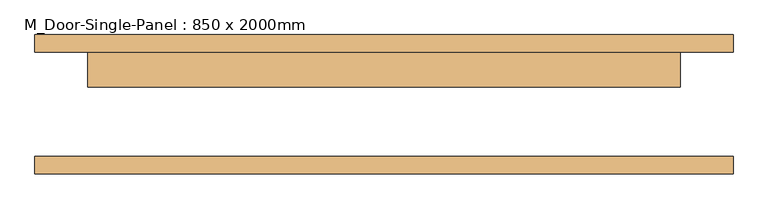
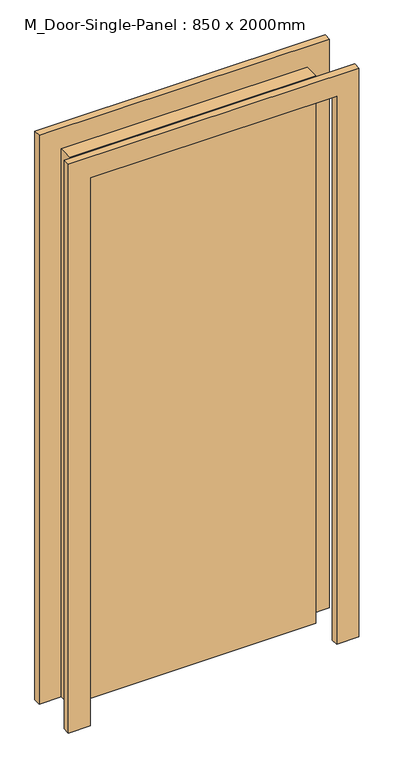
"""IFC4 building model written with IfcOpenShell, lengths in millimetres: door geometry, M_Door-Single-Panel : 850 x 2000mm."""

import ifcopenshell
import ifcopenshell.guid

model = None  # the IFC model being written
_history = None  # IfcOwnerHistory: only IFC2X3 demands one
_inside = {}  # id of a spatial element -> (the spatial element, [elements in it])
_under = {}  # id of a project, library or spatial element -> (it, [spatial elements below it])
_declared = {}  # id of a project -> (the project, [libraries it declares])
_typed = {}  # id of a type object -> (the type object, [elements of that type])
_made_of = {}  # id of a material, layer set ... -> (it, [elements and type objects made of it])


def new_model(schema):
    """Start an empty IFC model of exactly this schema.

    Asked for "IFC4X3", IfcOpenShell would pick the latest addendum, in which some entities
    have other attributes; the version numbers below select the first issue.
    IFC2X3 requires an IfcOwnerHistory on every rooted entity: one is made here for all.
    """
    global model, _history
    if schema == "IFC4X3":
        model = ifcopenshell.file(schema_version=(4, 3, 0, 0))
    else:
        model = ifcopenshell.file(schema=schema)
    _inside.clear()
    _under.clear()
    _declared.clear()
    _typed.clear()
    _made_of.clear()
    _history = None
    if model.schema == "IFC2X3":
        org = make("IfcOrganization", Name="unknown")
        user = make(
            "IfcPersonAndOrganization",
            ThePerson=make("IfcPerson", FamilyName="unknown"),
            TheOrganization=org,
        )
        app = make(
            "IfcApplication",
            ApplicationDeveloper=org,
            Version="unknown",
            ApplicationFullName="unknown",
            ApplicationIdentifier="unknown",
        )
        _history = make(
            "IfcOwnerHistory",
            OwningUser=user,
            OwningApplication=app,
            ChangeAction="ADDED",
            CreationDate=0,
        )
    return model


def make(cls, **values):
    """One entity of the class cls with the attributes given. An attribute that is None is left unset."""
    return model.create_entity(
        cls, **{name: value for name, value in values.items() if value is not None}
    )


def rooted(cls, **values):
    """An entity with a GlobalId (a new one), such as an element, a storey or a relation."""
    return make(cls, GlobalId=ifcopenshell.guid.new(), OwnerHistory=_history, **values)


def si_unit(unit_type, name, prefix=None):
    """IfcSIUnit, for example si_unit("LENGTHUNIT", "METRE", prefix="MILLI")."""
    return make("IfcSIUnit", UnitType=unit_type, Prefix=prefix, Name=name)


def assignment(units):
    """IfcUnitAssignment: the units of a project."""
    return None if units is None else make("IfcUnitAssignment", Units=units)


def point(xyz):
    """IfcCartesianPoint."""
    return None if xyz is None else make("IfcCartesianPoint", Coordinates=xyz)


def direction(xyz):
    """IfcDirection."""
    return None if xyz is None else make("IfcDirection", DirectionRatios=xyz)


def frame(location, z_axis=None, x_axis=None):
    """IfcAxis2Placement3D, a coordinate frame: its origin and axes. An axis left out is left unset."""
    return make(
        "IfcAxis2Placement3D",
        Location=point(location),
        Axis=direction(z_axis),
        RefDirection=direction(x_axis),
    )


def origin():
    """The frame at (0, 0, 0) with its axes left unset."""
    return frame((0.0, 0.0, 0.0))


def origin_with_axes():
    """The frame at (0, 0, 0) with the z axis (0, 0, 1) and the x axis (1, 0, 0) written out."""
    return frame((0.0, 0.0, 0.0), z_axis=(0.0, 0.0, 1.0), x_axis=(1.0, 0.0, 0.0))


def place(relative_to, where):
    """IfcLocalPlacement: puts the frame where relative to a parent placement (None: the world)."""
    return make(
        "IfcLocalPlacement", PlacementRelTo=relative_to, RelativePlacement=where
    )


def context(
    kind, dimensions, precision=None, world=None, true_north=None, identifier=None
):
    """IfcGeometricRepresentationContext, for example the 3D "Model" context."""
    return make(
        "IfcGeometricRepresentationContext",
        ContextIdentifier=identifier,
        ContextType=kind,
        CoordinateSpaceDimension=dimensions,
        Precision=precision,
        WorldCoordinateSystem=world,
        TrueNorth=true_north,
    )


def project(units=None, contexts=None):
    """IfcProject with its units and contexts."""
    return rooted(
        "IfcProject",
        Name="project",
        RepresentationContexts=contexts,
        UnitsInContext=assignment(units),
    )


def spatial(cls, under=None, at=None, **own):
    """A site, building, storey or space (cls), placed at a placement, below another one or the project."""
    s = rooted(cls, ObjectPlacement=at, **own)
    if under is not None:
        _under.setdefault(under.id(), (under, []))[1].append(s)
    return s


def polyline(points):
    """IfcPolyline through the points."""
    return make("IfcPolyline", Points=[point(p) for p in points])


def outline(outer, holes=None, kind="AREA"):
    """IfcArbitraryClosedProfileDef: a profile drawn as a closed curve; with holes, ...WithVoids."""
    if holes is None:
        return make("IfcArbitraryClosedProfileDef", ProfileType=kind, OuterCurve=outer)
    return make(
        "IfcArbitraryProfileDefWithVoids",
        ProfileType=kind,
        OuterCurve=outer,
        InnerCurves=holes,
    )


def extrude(swept, where, along, depth):
    """IfcExtrudedAreaSolid: the profile swept, set in the frame where, extruded along a direction by depth."""
    return make(
        "IfcExtrudedAreaSolid",
        SweptArea=swept,
        Position=where,
        ExtrudedDirection=direction(along),
        Depth=depth,
    )


def shape(context_of_items, identifier, shape_type, items):
    """IfcShapeRepresentation: the items that make up one representation, for example the "Body"."""
    return make(
        "IfcShapeRepresentation",
        ContextOfItems=context_of_items,
        RepresentationIdentifier=identifier,
        RepresentationType=shape_type,
        Items=items,
    )


def source(mapping_origin, context_of_items, identifier, shape_type, items):
    """IfcRepresentationMap: a shape defined once, which mapped items show again and again."""
    return make(
        "IfcRepresentationMap",
        MappingOrigin=mapping_origin,
        MappedRepresentation=shape(context_of_items, identifier, shape_type, items),
    )


def transform(
    local_origin,
    x_axis=None,
    y_axis=None,
    z_axis=None,
    scale=None,
    scale2=None,
    scale3=None,
    uniform=True,
):
    """IfcCartesianTransformationOperator3D, or its non-uniform kind. x_axis, y_axis, z_axis: its Axis1, 2, 3."""
    if uniform:
        return make(
            "IfcCartesianTransformationOperator3D",
            Axis1=direction(x_axis),
            Axis2=direction(y_axis),
            LocalOrigin=point(local_origin),
            Scale=scale,
            Axis3=direction(z_axis),
        )
    return make(
        "IfcCartesianTransformationOperator3DnonUniform",
        Axis1=direction(x_axis),
        Axis2=direction(y_axis),
        LocalOrigin=point(local_origin),
        Scale=scale,
        Axis3=direction(z_axis),
        Scale2=scale2,
        Scale3=scale3,
    )


def mapped(mapping_source, mapping_target):
    """IfcMappedItem: shows the shape of a source again, moved by a transform."""
    return make(
        "IfcMappedItem", MappingSource=mapping_source, MappingTarget=mapping_target
    )


def made_of(thing, what):
    """Note that an element or type object is made of a material, layer set ...; save() writes the relation."""
    if what is not None:
        _made_of.setdefault(what.id(), (what, []))[1].append(thing)
    return thing


def element(
    cls,
    number,
    at=None,
    inside=None,
    cuts=None,
    type_object=None,
    material=None,
    context=None,
    identifier="Body",
    shape_type=None,
    held_by="IfcProductDefinitionShape",
    body=None,
    shapes=None,
    **own,
):
    """One element of the class cls, such as IfcWall. Its Tag is "e" and its number.

    at: its placement. inside: the storey or other place that contains it. cuts: it is an
    opening in that element (IfcRelVoidsElement). A single representation is given by context,
    identifier, shape_type and body (its items); several are given by shapes. held_by: the class
    of the entity that holds the representations. save() writes the other relations.
    """
    e = rooted(cls, Tag="e%d" % number, ObjectPlacement=at, **own)
    if body is not None:
        shapes = [shape(context, identifier, shape_type, body)]
    if shapes is not None:
        e.Representation = make(held_by, Representations=shapes)
    if inside is not None:
        _inside.setdefault(inside.id(), (inside, []))[1].append(e)
    if cuts is not None:
        rooted(
            "IfcRelVoidsElement", RelatingBuildingElement=cuts, RelatedOpeningElement=e
        )
    if type_object is not None:
        _typed.setdefault(type_object.id(), (type_object, []))[1].append(e)
    return made_of(e, material)


def aggregate(whole, parts):
    """IfcRelAggregates: a whole, such as a stair, and the parts it consists of."""
    return rooted("IfcRelAggregates", RelatingObject=whole, RelatedObjects=parts)


def save(model, path):
    """Write the relations noted so far, then the file.

    IfcRelAggregates (storeys below a building ...), IfcRelContainedInSpatialStructure (elements
    in a storey), IfcRelDefinesByType, IfcRelAssociatesMaterial and IfcRelDeclares: one each for
    every whole, place, type object, material and project.
    """
    for whole, parts in _under.values():
        aggregate(whole, parts)
    for where, things in _inside.values():
        rooted(
            "IfcRelContainedInSpatialStructure",
            RelatedElements=things,
            RelatingStructure=where,
        )
    for kind, things in _typed.values():
        rooted("IfcRelDefinesByType", RelatedObjects=things, RelatingType=kind)
    for what, things in _made_of.values():
        rooted("IfcRelAssociatesMaterial", RelatedObjects=things, RelatingMaterial=what)
    for by, libraries in _declared.values():
        rooted("IfcRelDeclares", RelatingContext=by, RelatedDefinitions=libraries)
    model.write(path)


def m_door_single_panel_850_x_2000mm_c4dca14f(model_context):
    return source(origin(), model_context, "Body", "SweptSolid", [
        extrude(outline(polyline([(425.0, 25.0), (-425.0, 25.0), (-425.0, 75.0), (425.0, 75.0), (425.0, 25.0)])), origin_with_axes(), (0.0, 0.0, 1.0), 2000.0),
        extrude(outline(polyline([(2076.2, -501.2), (0.0, -501.2), (0.0, -425.0), (2000.0, -425.0), (2000.0, 425.0), (0.0, 425.0), (0.0, 501.2), (2076.2, 501.2), (2076.2, -501.2)])), frame((0.0, 75.0, 0.0), z_axis=(0.0, 1.0, 0.0), x_axis=(0.0, 0.0, 1.0)), (0.0, 0.0, 1.0), 25.0),
        extrude(outline(polyline([(2076.2, 501.2), (2076.2, -501.2), (0.0, -501.2), (0.0, -425.0), (2000.0, -425.0), (2000.0, 425.0), (0.0, 425.0), (0.0, 501.2), (2076.2, 501.2)])), frame((0.0, -100.0, 0.0), z_axis=(0.0, 1.0, 0.0), x_axis=(0.0, 0.0, 1.0)), (0.0, 0.0, 1.0), 25.0),
    ])


if __name__ == "__main__":
    model = new_model("IFC4")
    model_context = context("Model", 3, world=origin())
    ifc_project = project(units=[si_unit("LENGTHUNIT", "METRE", prefix="MILLI")], contexts=[model_context])
    site = spatial("IfcSite", under=ifc_project)
    building = spatial("IfcBuilding", under=site)
    placement = place(None, origin())
    m_door_single_panel_850_x_2000mm_shape = m_door_single_panel_850_x_2000mm_c4dca14f(model_context)
    element("IfcDoor", 1, ObjectType="M_Door-Single-Panel : 850 x 2000mm", at=placement, inside=building, context=model_context, shape_type="MappedRepresentation", body=[
        mapped(m_door_single_panel_850_x_2000mm_shape, transform((0.0, 0.0, 0.0), x_axis=(1.0, 0.0, 0.0), y_axis=(0.0, 1.0, 0.0), z_axis=(0.0, 0.0, 1.0))),
    ])
    save(model, "model.ifc")

# Revit data of these elements
# Type "M_Door-Single-Panel : 850 x 2000mm"
#   Type Mark = "23"
#   Construction Type Id = "DOOR"
#   Assembly Code = "C1020300"
#   Analytic Construction = "Wooden"
#   Thickness = 0.05 m
#   Thermal Resistance (R) = 0.455703 (m²·K)/W
#   Swing Angle [instance default] = 90.00°
#   Heat Transfer Coefficient (U) = 2.19465 W/(m²·K)
#   Height = 2 m
#   Trim Projection Ext = 0.025 m
#   Trim Projection Int = 0.025 m
#   Trim Width = 0.08 m
#   Width = 0.85 m
#   Panel Material = Wood - Birch - Solid Stained Light Low Gloss
#   Trim Material = Paint - Sienna
#   Visual Light Transmittance = 0
#   Solar Heat Gain Coefficient = 0
#   Function = (empty or 0)
#   Wall Closure = (empty or 0)
# Element 1 (IfcDoor, "M_Door-Single-Panel : 850 x 2000mm")
#   Materials on its faces: "Paint - Sienna", "Wood - Birch - Solid Stained Light Low Gloss"
# Materials
#   "Wood - Birch - Solid Stained Light Low Gloss": class "Wood", colour RGB 227 170 128, transparency 0, Cost = 0
#   "Paint - Sienna": class "Miscellaneous", colour RGB 118 70 51, transparency 0, Cost = 0
